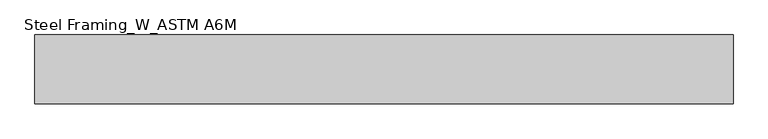
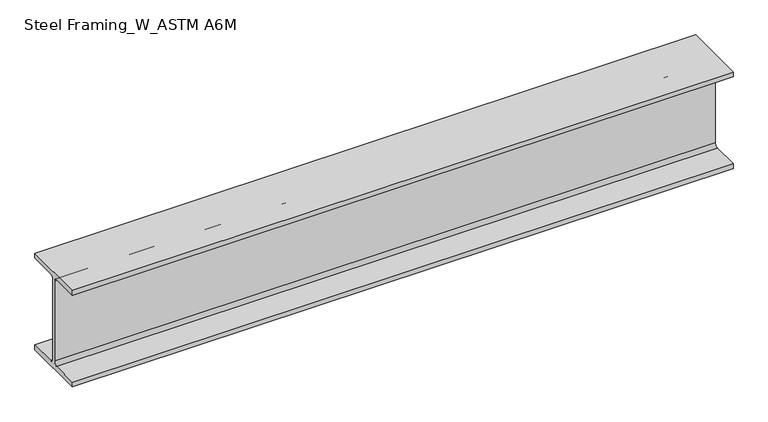
"""IFC4 building model written with IfcOpenShell, lengths in millimetres: beam geometry, Steel Framing_W_ASTM A6M : H_SB_AR_S02_W200x31.3_B6."""

from ifc_helpers import new_model, si_unit, point, frame, frame_2d, origin, place, context, project, spatial, polyline, circle_curve, trimmed, segment, composite_curve, outline, extrude, source, transform, mapped, element, save


def steel_framing_w_astm_a6m_e50dfa28(model_context):
    return source(origin(), model_context, "Body", "SweptSolid", [
        extrude(outline(composite_curve([segment(polyline([(67.0, -94.8), (67.0, -105.0), (-67.0, -105.0), (-67.0, -94.8), (-10.775, -94.8)]), True, "CONTINUOUS"), segment(trimmed(circle_curve(frame_2d((-10.775, -87.2)), 7.6), [point((-10.775, -94.8))], [point((-3.175, -87.2))], True, "CARTESIAN"), True, "CONTINUOUS"), segment(polyline([(-3.175, -87.2), (-3.175, 87.2)]), True, "CONTINUOUS"), segment(trimmed(circle_curve(frame_2d((-10.775, 87.2)), 7.6), [point((-3.175, 87.2))], [point((-10.775, 94.8))], True, "CARTESIAN"), True, "CONTINUOUS"), segment(polyline([(-10.775, 94.8), (-67.0, 94.8), (-67.0, 105.0), (67.0, 105.0), (67.0, 94.8), (10.775, 94.8)]), True, "CONTINUOUS"), segment(trimmed(circle_curve(frame_2d((10.775, 87.2)), 7.6), [point((10.775, 94.8))], [point((3.175, 87.2))], True, "CARTESIAN"), True, "CONTINUOUS"), segment(polyline([(3.175, 87.2), (3.175, -87.2)]), True, "CONTINUOUS"), segment(trimmed(circle_curve(frame_2d((10.775, -87.2)), 7.6), [point((3.175, -87.2))], [point((10.775, -94.8))], True, "CARTESIAN"), True, "CONTINUOUS"), segment(polyline([(10.775, -94.8), (67.0, -94.8)]), True, "CONTINUOUS")], self_intersect=False)), frame((-660.3, 0.0, 0.0), z_axis=(1.0, 0.0, 0.0), x_axis=(0.0, 1.0, 0.0)), (0.0, 0.0, 1.0), 1362.1),
    ])


if __name__ == "__main__":
    model = new_model("IFC4")
    model_context = context("Model", 3, world=origin())
    ifc_project = project(units=[si_unit("LENGTHUNIT", "METRE", prefix="MILLI")], contexts=[model_context])
    site = spatial("IfcSite", under=ifc_project)
    building = spatial("IfcBuilding", under=site)
    placement = place(None, origin())
    steel_framing_w_astm_a6m_shape = steel_framing_w_astm_a6m_e50dfa28(model_context)
    element("IfcBeam", 1, ObjectType="Steel Framing_W_ASTM A6M : H_SB_AR_S02_W200x31.3_B6", at=placement, inside=building, context=model_context, shape_type="MappedRepresentation", body=[
        mapped(steel_framing_w_astm_a6m_shape, transform((0.0, 0.0, 0.0), x_axis=(1.0, 0.0, 0.0), y_axis=(0.0, 1.0, 0.0), z_axis=(0.0, 0.0, 1.0))),
    ])
    save(model, "model.ifc")

# Revit data of these elements
# Type "Steel Framing_W_ASTM A6M : H_SB_AR_S02_W200x31.3_B6"
#   Type Mark = "B6"
#   Section Name Key = "W8x21"
#   Width = 13.4 cm
#   Web Thickness = 0.635 cm
#   Web Fillet = 0.76 cm
#   Warping Constant = 40800.0 cm⁶
#   Torsional Moment of Inertia = 11.70 cm⁴
#   Section Area = 39.7 cm²
#   Plastic Modulus weak axis = 93.2 cm³
#   Plastic Modulus strong axis = 334.0 cm³
#   Perimeter = 0.93 m²/m
#   Nominal Weight = 31.30 kgf/m
#   Moment of Inertia weak axis = 407.00 cm⁴
#   Moment of Inertia strong axis = 3130.00 cm⁴
#   Height = 21.0 cm
#   Flange Thickness = 1.02 cm
#   Elastic Modulus weak axis = 60.8 cm³
#   Elastic Modulus strong axis = 298.0 cm³
#   Centroid Vertical = 10.5 cm
#   Centroid Horizontal = 6.7 cm
#   Length [instance default] = 1500 mm
#   Structural Material [instance default] = Steel, 45-345
#   Bolt Spacing = 0
#   Assembly Code = ""
# Element 1 (IfcBeam, "Steel Framing_W_ASTM A6M : H_SB_AR_S02_W200x31.3_B6")
#   Materials on its faces: "Steel, 45-345"
# Materials
#   "Steel, 45-345": class "Metal", colour RGB 189 187 185, transparency 0, Description = "Steel 345 MPa", Cost = 0
